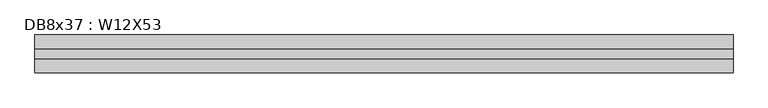
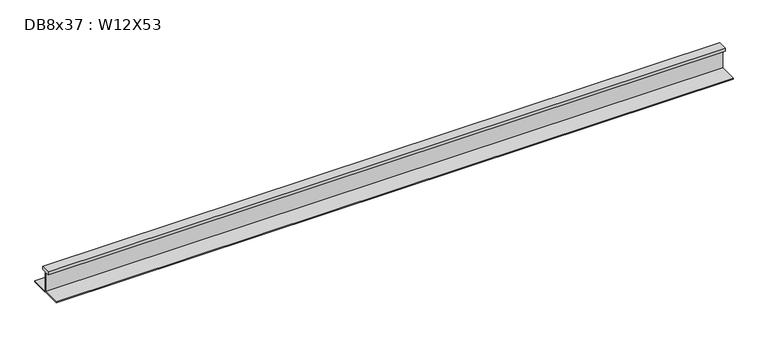
"""IFC4 building model written with IfcOpenShell, lengths in millimetres: beam geometry, DB8x37 : W12X53."""

import ifcopenshell
import ifcopenshell.guid

model = None  # the IFC model being written
_history = None  # IfcOwnerHistory: only IFC2X3 demands one
_inside = {}  # id of a spatial element -> (the spatial element, [elements in it])
_under = {}  # id of a project, library or spatial element -> (it, [spatial elements below it])
_declared = {}  # id of a project -> (the project, [libraries it declares])
_typed = {}  # id of a type object -> (the type object, [elements of that type])
_made_of = {}  # id of a material, layer set ... -> (it, [elements and type objects made of it])


def new_model(schema):
    """Start an empty IFC model of exactly this schema.

    Asked for "IFC4X3", IfcOpenShell would pick the latest addendum, in which some entities
    have other attributes; the version numbers below select the first issue.
    IFC2X3 requires an IfcOwnerHistory on every rooted entity: one is made here for all.
    """
    global model, _history
    if schema == "IFC4X3":
        model = ifcopenshell.file(schema_version=(4, 3, 0, 0))
    else:
        model = ifcopenshell.file(schema=schema)
    _inside.clear()
    _under.clear()
    _declared.clear()
    _typed.clear()
    _made_of.clear()
    _history = None
    if model.schema == "IFC2X3":
        org = make("IfcOrganization", Name="unknown")
        user = make(
            "IfcPersonAndOrganization",
            ThePerson=make("IfcPerson", FamilyName="unknown"),
            TheOrganization=org,
        )
        app = make(
            "IfcApplication",
            ApplicationDeveloper=org,
            Version="unknown",
            ApplicationFullName="unknown",
            ApplicationIdentifier="unknown",
        )
        _history = make(
            "IfcOwnerHistory",
            OwningUser=user,
            OwningApplication=app,
            ChangeAction="ADDED",
            CreationDate=0,
        )
    return model


def make(cls, **values):
    """One entity of the class cls with the attributes given. An attribute that is None is left unset."""
    return model.create_entity(
        cls, **{name: value for name, value in values.items() if value is not None}
    )


def rooted(cls, **values):
    """An entity with a GlobalId (a new one), such as an element, a storey or a relation."""
    return make(cls, GlobalId=ifcopenshell.guid.new(), OwnerHistory=_history, **values)


def si_unit(unit_type, name, prefix=None):
    """IfcSIUnit, for example si_unit("LENGTHUNIT", "METRE", prefix="MILLI")."""
    return make("IfcSIUnit", UnitType=unit_type, Prefix=prefix, Name=name)


def assignment(units):
    """IfcUnitAssignment: the units of a project."""
    return None if units is None else make("IfcUnitAssignment", Units=units)


def point(xyz):
    """IfcCartesianPoint."""
    return None if xyz is None else make("IfcCartesianPoint", Coordinates=xyz)


def direction(xyz):
    """IfcDirection."""
    return None if xyz is None else make("IfcDirection", DirectionRatios=xyz)


def frame(location, z_axis=None, x_axis=None):
    """IfcAxis2Placement3D, a coordinate frame: its origin and axes. An axis left out is left unset."""
    return make(
        "IfcAxis2Placement3D",
        Location=point(location),
        Axis=direction(z_axis),
        RefDirection=direction(x_axis),
    )


def origin():
    """The frame at (0, 0, 0) with its axes left unset."""
    return frame((0.0, 0.0, 0.0))


def place(relative_to, where):
    """IfcLocalPlacement: puts the frame where relative to a parent placement (None: the world)."""
    return make(
        "IfcLocalPlacement", PlacementRelTo=relative_to, RelativePlacement=where
    )


def context(
    kind, dimensions, precision=None, world=None, true_north=None, identifier=None
):
    """IfcGeometricRepresentationContext, for example the 3D "Model" context."""
    return make(
        "IfcGeometricRepresentationContext",
        ContextIdentifier=identifier,
        ContextType=kind,
        CoordinateSpaceDimension=dimensions,
        Precision=precision,
        WorldCoordinateSystem=world,
        TrueNorth=true_north,
    )


def project(units=None, contexts=None):
    """IfcProject with its units and contexts."""
    return rooted(
        "IfcProject",
        Name="project",
        RepresentationContexts=contexts,
        UnitsInContext=assignment(units),
    )


def spatial(cls, under=None, at=None, **own):
    """A site, building, storey or space (cls), placed at a placement, below another one or the project."""
    s = rooted(cls, ObjectPlacement=at, **own)
    if under is not None:
        _under.setdefault(under.id(), (under, []))[1].append(s)
    return s


def polyline(points):
    """IfcPolyline through the points."""
    return make("IfcPolyline", Points=[point(p) for p in points])


def outline(outer, holes=None, kind="AREA"):
    """IfcArbitraryClosedProfileDef: a profile drawn as a closed curve; with holes, ...WithVoids."""
    if holes is None:
        return make("IfcArbitraryClosedProfileDef", ProfileType=kind, OuterCurve=outer)
    return make(
        "IfcArbitraryProfileDefWithVoids",
        ProfileType=kind,
        OuterCurve=outer,
        InnerCurves=holes,
    )


def extrude(swept, where, along, depth):
    """IfcExtrudedAreaSolid: the profile swept, set in the frame where, extruded along a direction by depth."""
    return make(
        "IfcExtrudedAreaSolid",
        SweptArea=swept,
        Position=where,
        ExtrudedDirection=direction(along),
        Depth=depth,
    )


def shape(context_of_items, identifier, shape_type, items):
    """IfcShapeRepresentation: the items that make up one representation, for example the "Body"."""
    return make(
        "IfcShapeRepresentation",
        ContextOfItems=context_of_items,
        RepresentationIdentifier=identifier,
        RepresentationType=shape_type,
        Items=items,
    )


def source(mapping_origin, context_of_items, identifier, shape_type, items):
    """IfcRepresentationMap: a shape defined once, which mapped items show again and again."""
    return make(
        "IfcRepresentationMap",
        MappingOrigin=mapping_origin,
        MappedRepresentation=shape(context_of_items, identifier, shape_type, items),
    )


def transform(
    local_origin,
    x_axis=None,
    y_axis=None,
    z_axis=None,
    scale=None,
    scale2=None,
    scale3=None,
    uniform=True,
):
    """IfcCartesianTransformationOperator3D, or its non-uniform kind. x_axis, y_axis, z_axis: its Axis1, 2, 3."""
    if uniform:
        return make(
            "IfcCartesianTransformationOperator3D",
            Axis1=direction(x_axis),
            Axis2=direction(y_axis),
            LocalOrigin=point(local_origin),
            Scale=scale,
            Axis3=direction(z_axis),
        )
    return make(
        "IfcCartesianTransformationOperator3DnonUniform",
        Axis1=direction(x_axis),
        Axis2=direction(y_axis),
        LocalOrigin=point(local_origin),
        Scale=scale,
        Axis3=direction(z_axis),
        Scale2=scale2,
        Scale3=scale3,
    )


def mapped(mapping_source, mapping_target):
    """IfcMappedItem: shows the shape of a source again, moved by a transform."""
    return make(
        "IfcMappedItem", MappingSource=mapping_source, MappingTarget=mapping_target
    )


def made_of(thing, what):
    """Note that an element or type object is made of a material, layer set ...; save() writes the relation."""
    if what is not None:
        _made_of.setdefault(what.id(), (what, []))[1].append(thing)
    return thing


def element(
    cls,
    number,
    at=None,
    inside=None,
    cuts=None,
    type_object=None,
    material=None,
    context=None,
    identifier="Body",
    shape_type=None,
    held_by="IfcProductDefinitionShape",
    body=None,
    shapes=None,
    **own,
):
    """One element of the class cls, such as IfcWall. Its Tag is "e" and its number.

    at: its placement. inside: the storey or other place that contains it. cuts: it is an
    opening in that element (IfcRelVoidsElement). A single representation is given by context,
    identifier, shape_type and body (its items); several are given by shapes. held_by: the class
    of the entity that holds the representations. save() writes the other relations.
    """
    e = rooted(cls, Tag="e%d" % number, ObjectPlacement=at, **own)
    if body is not None:
        shapes = [shape(context, identifier, shape_type, body)]
    if shapes is not None:
        e.Representation = make(held_by, Representations=shapes)
    if inside is not None:
        _inside.setdefault(inside.id(), (inside, []))[1].append(e)
    if cuts is not None:
        rooted(
            "IfcRelVoidsElement", RelatingBuildingElement=cuts, RelatedOpeningElement=e
        )
    if type_object is not None:
        _typed.setdefault(type_object.id(), (type_object, []))[1].append(e)
    return made_of(e, material)


def aggregate(whole, parts):
    """IfcRelAggregates: a whole, such as a stair, and the parts it consists of."""
    return rooted("IfcRelAggregates", RelatingObject=whole, RelatedObjects=parts)


def save(model, path):
    """Write the relations noted so far, then the file.

    IfcRelAggregates (storeys below a building ...), IfcRelContainedInSpatialStructure (elements
    in a storey), IfcRelDefinesByType, IfcRelAssociatesMaterial and IfcRelDeclares: one each for
    every whole, place, type object, material and project.
    """
    for whole, parts in _under.values():
        aggregate(whole, parts)
    for where, things in _inside.values():
        rooted(
            "IfcRelContainedInSpatialStructure",
            RelatedElements=things,
            RelatingStructure=where,
        )
    for kind, things in _typed.values():
        rooted("IfcRelDefinesByType", RelatedObjects=things, RelatingType=kind)
    for what, things in _made_of.values():
        rooted("IfcRelAssociatesMaterial", RelatedObjects=things, RelatingMaterial=what)
    for by, libraries in _declared.values():
        rooted("IfcRelDeclares", RelatingContext=by, RelatedDefinitions=libraries)
    model.write(path)


def db8x37_w12x53_1dfed5d5(model_context):
    return source(origin(), model_context, "Body", "SweptSolid", [
        extrude(outline(polyline([(38.1, 145.415), (38.1, 120.015), (2.921, 120.015), (2.921, -48.4505), (152.4, -48.4505), (152.4, -58.1025), (-152.4, -58.1025), (-152.4, -48.4505), (-2.921, -48.4505), (-2.921, 120.015), (-38.1, 120.015), (-38.1, 145.415), (38.1, 145.415)])), frame((-2878.8042219, 0.0, 0.0), z_axis=(1.0, 0.0, 0.0), x_axis=(0.0, 1.0, 0.0)), (0.0, 0.0, 1.0), 5601.668375),
    ])


if __name__ == "__main__":
    model = new_model("IFC4")
    model_context = context("Model", 3, world=origin())
    ifc_project = project(units=[si_unit("LENGTHUNIT", "METRE", prefix="MILLI")], contexts=[model_context])
    site = spatial("IfcSite", under=ifc_project)
    building = spatial("IfcBuilding", under=site)
    placement = place(None, origin())
    db8x37_w12x53_shape = db8x37_w12x53_1dfed5d5(model_context)
    element("IfcBeam", 1, ObjectType="DB8x37 : W12X53", at=placement, inside=building, context=model_context, shape_type="MappedRepresentation", body=[
        mapped(db8x37_w12x53_shape, transform((0.0, 0.0, 0.0), x_axis=(1.0, 0.0, 0.0), y_axis=(0.0, 1.0, 0.0), z_axis=(0.0, 0.0, 1.0))),
    ])
    save(model, "model.ifc")

# Revit data of these elements
# Type "DB8x37 : W12X53"
#   Assembly Code = "B10"
#   W = 53
#   Length [instance default] = 5' - 0"
#   bf = 0' - 10"
#   d = 1' - 0.1"
#   k = 0' - 1 3/8"
#   k2 = 0' - 0.8"
#   tf = 0' - 0.575"
#   tw = 0' - 0.345"
#   A = 0.108333 SF
#   Structural Material [instance default] = Steel ASTM A992
# Element 1 (IfcBeam, "DB8x37 : W12X53")
#   Materials on its faces: "Steel ASTM A992"
# Materials
#   "Steel ASTM A992": class "Metal", colour RGB 199 199 199, transparency 0, Description = "Structural steel 50ksi", Cost = 0
